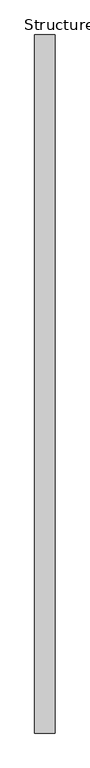
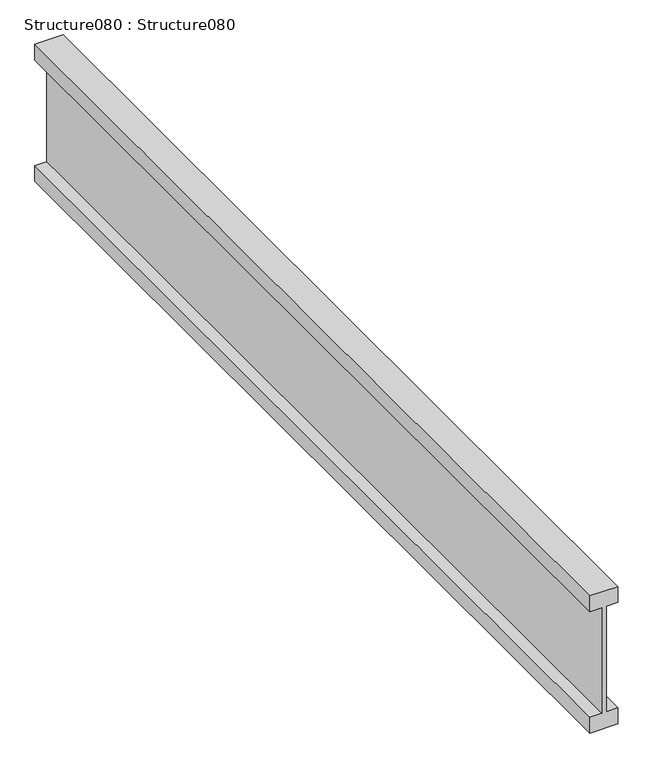
"""IFC4 building model written with IfcOpenShell, lengths in millimetres: proxy geometry, Structure080 : Structure080."""

from ifc_helpers import new_model, si_unit, frame, origin, place, context, project, spatial, polyline, outline, extrude, source, transform, mapped, element, save


def structure080_structure080_4a0a86c5(model_context):
    return source(origin(), model_context, "Body", "SweptSolid", [
        extrude(outline(polyline([(36420.171, -2811.6168586), (36420.171, -2787.0106086), (36188.396, -2787.0106086), (36188.396, -2811.6168586), (36153.471, -2811.6168586), (36153.471, -2752.8793586), (36188.396, -2752.8793586), (36188.396, -2777.4856086), (36420.171, -2777.4856086), (36420.171, -2752.8793586), (36455.096, -2752.8793586), (36455.096, -2811.6168586), (36420.171, -2811.6168586)])), frame((0.0, 998.1570053, 0.0), z_axis=(0.0, 1.0, 0.0), x_axis=(0.0, 0.0, 1.0)), (0.0, 0.0, 1.0), 2000.0),
    ])


if __name__ == "__main__":
    model = new_model("IFC4")
    model_context = context("Model", 3, world=origin())
    ifc_project = project(units=[si_unit("LENGTHUNIT", "METRE", prefix="MILLI")], contexts=[model_context])
    site = spatial("IfcSite", under=ifc_project)
    building = spatial("IfcBuilding", under=site)
    placement = place(None, origin())
    structure080_structure080_shape = structure080_structure080_4a0a86c5(model_context)
    element("IfcBuildingElementProxy", 1, Name="Structure080 : Structure080", ObjectType="Structure080 : Structure080", at=placement, inside=building, context=model_context, shape_type="MappedRepresentation", body=[
        mapped(structure080_structure080_shape, transform((0.0, 0.0, 0.0), x_axis=(1.0, 0.0, 0.0), y_axis=(0.0, 1.0, 0.0), z_axis=(0.0, 0.0, 1.0))),
    ])
    save(model, "model.ifc")

# Revit data of these elements
# Type "Structure080 : Structure080"
#   NameOverride = "Structure080"
# Element 1 (IfcBuildingElementProxy, "Structure080 : Structure080")
#   Materials on its faces: "WOOD FRAMING (SEE STRUCT DWGS)"
# Materials
#   "WOOD FRAMING (SEE STRUCT DWGS)": class "Unassigned", colour RGB 224 188 168, transparency 0, Cost = 0
